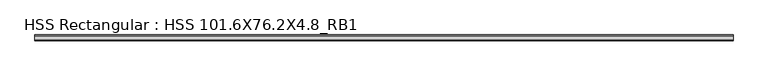
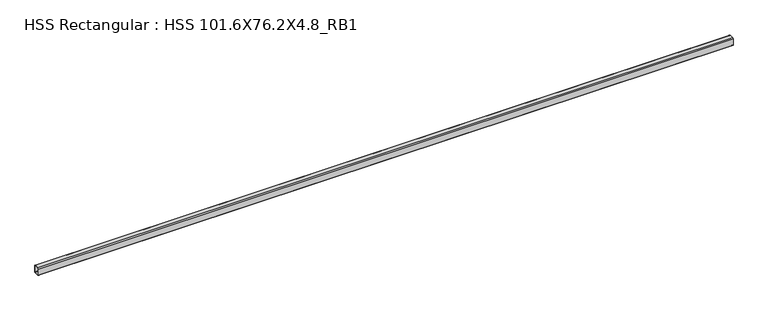
"""IFC4 building model written with IfcOpenShell, lengths in millimetres: beam geometry, HSS Rectangular : HSS 101.6X76.2X4.8_RB1."""

from ifc_helpers import new_model, si_unit, point, frame, frame_2d, origin, place, context, project, spatial, polyline, circle_curve, trimmed, segment, composite_curve, outline, extrude, source, transform, mapped, element, save


def hss_rectangular_hss_101_6x76_2x4_8_rb1_cf643c91(model_context):
    return source(origin(), model_context, "Body", "SweptSolid", [
        extrude(outline(composite_curve([segment(trimmed(circle_curve(frame_2d((-28.575, 41.275)), 9.525), [point((-38.1, 41.275))], [point((-28.575, 50.8))], False, "CARTESIAN"), True, "CONTINUOUS"), segment(polyline([(-28.575, 50.8), (28.575, 50.8)]), True, "CONTINUOUS"), segment(trimmed(circle_curve(frame_2d((28.575, 41.275)), 9.525), [point((28.575, 50.8))], [point((38.1, 41.275))], False, "CARTESIAN"), True, "CONTINUOUS"), segment(polyline([(38.1, 41.275), (38.1, -41.275)]), True, "CONTINUOUS"), segment(trimmed(circle_curve(frame_2d((28.575, -41.275)), 9.525), [point((38.1, -41.275))], [point((28.575, -50.8))], False, "CARTESIAN"), True, "CONTINUOUS"), segment(polyline([(28.575, -50.8), (-28.575, -50.8)]), True, "CONTINUOUS"), segment(trimmed(circle_curve(frame_2d((-28.575, -41.275)), 9.525), [point((-28.575, -50.8))], [point((-38.1, -41.275))], False, "CARTESIAN"), True, "CONTINUOUS"), segment(polyline([(-38.1, -41.275), (-38.1, 41.275)]), True, "CONTINUOUS")], self_intersect=False), holes=[composite_curve([segment(polyline([(28.575, 46.0375), (-28.575, 46.0375)]), True, "CONTINUOUS"), segment(trimmed(circle_curve(frame_2d((-28.575, 41.275)), 4.7625), [point((-28.575, 46.0375))], [point((-33.3375, 41.275))], True, "CARTESIAN"), True, "CONTINUOUS"), segment(polyline([(-33.3375, 41.275), (-33.3375, -41.275)]), True, "CONTINUOUS"), segment(trimmed(circle_curve(frame_2d((-28.575, -41.275)), 4.7625), [point((-33.3375, -41.275))], [point((-28.575, -46.0375))], True, "CARTESIAN"), True, "CONTINUOUS"), segment(polyline([(-28.575, -46.0375), (28.575, -46.0375)]), True, "CONTINUOUS"), segment(trimmed(circle_curve(frame_2d((28.575, -41.275)), 4.7625), [point((28.575, -46.0375))], [point((33.3375, -41.275))], True, "CARTESIAN"), True, "CONTINUOUS"), segment(polyline([(33.3375, -41.275), (33.3375, 41.275)]), True, "CONTINUOUS"), segment(trimmed(circle_curve(frame_2d((28.575, 41.275)), 4.7625), [point((33.3375, 41.275))], [point((28.575, 46.0375))], True, "CARTESIAN"), True, "CONTINUOUS")], self_intersect=False)]), frame((-7490.0, 0.0, 0.0), z_axis=(1.0, 0.0, 0.0), x_axis=(0.0, 1.0, 0.0)), (0.0, 0.0, 1.0), 8990.0),
    ])


if __name__ == "__main__":
    model = new_model("IFC4")
    model_context = context("Model", 3, world=origin())
    ifc_project = project(units=[si_unit("LENGTHUNIT", "METRE", prefix="MILLI")], contexts=[model_context])
    site = spatial("IfcSite", under=ifc_project)
    building = spatial("IfcBuilding", under=site)
    placement = place(None, origin())
    hss_rectangular_hss_101_6x76_2x4_8_rb1_shape = hss_rectangular_hss_101_6x76_2x4_8_rb1_cf643c91(model_context)
    element("IfcBeam", 1, ObjectType="HSS Rectangular : HSS 101.6X76.2X4.8_RB1", at=placement, inside=building, context=model_context, shape_type="MappedRepresentation", body=[
        mapped(hss_rectangular_hss_101_6x76_2x4_8_rb1_shape, transform((0.0, 0.0, 0.0), x_axis=(1.0, 0.0, 0.0), y_axis=(0.0, 1.0, 0.0), z_axis=(0.0, 0.0, 1.0))),
    ])
    save(model, "model.ifc")

# Revit data of these elements
# Type "HSS Rectangular : HSS 101.6X76.2X4.8_RB1"
#   Section Name Key = "HSS 4X3X3/16"
#   Assembly Code = "B10"
#   Width = 7.62 cm
#   Wall Nominal Thickness = 0.4763 cm
#   Wall Design Thickness = 0.442 cm
#   Torsional Moment of Inertia = 260.561 cm⁴
#   Torsional Modulus = 61.2876 cm³
#   Section Area = 14.4516 cm²
#   Plastic Modulus weak axis = 40.3122 cm³
#   Plastic Modulus strong axis = 49.1612 cm³
#   Perimeter = 0.881482 m²/m
#   Outer Fillet = 0.9525 cm
#   Nominal Weight = 12.1285 kgf/m
#   Moment of Inertia weak axis = 131.529 cm⁴
#   Moment of Inertia strong axis = 205.202 cm⁴
#   Inner Fillet = 0.4763 cm
#   Height = 10.16 cm
#   Elastic Modulus weak axis = 34.4128 cm³
#   Elastic Modulus strong axis = 40.476 cm³
#   Centroid Vertical = 5.08 cm
#   Centroid Horizontal = 3.81 cm
#   Length [instance default] = 1524 mm
#   Structural Material [instance default] = Steel ASTM A500, Grade B, Rectangular and Square
#   Principal Axes Angle = 0
# Element 1 (IfcBeam, "HSS Rectangular : HSS 101.6X76.2X4.8_RB1")
#   Structural Material = Steel ASTM A992
#   Materials on its faces: "Steel ASTM A992"
# Materials
#   "Steel ASTM A500, Grade B, Rectangular and Square": class "Metal", colour RGB 199 199 199, transparency 0, Description = "Carbon steel", Cost = 0
#   "Steel ASTM A992": class "Metal", colour RGB 199 199 199, transparency 0, Description = "Structural steel 50ksi", Cost = 0
